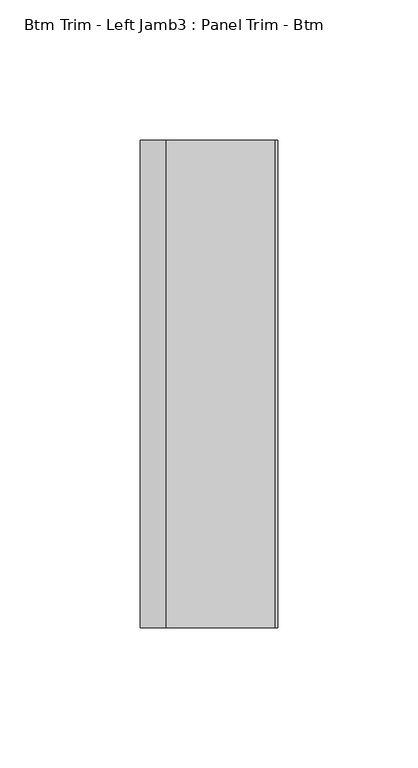
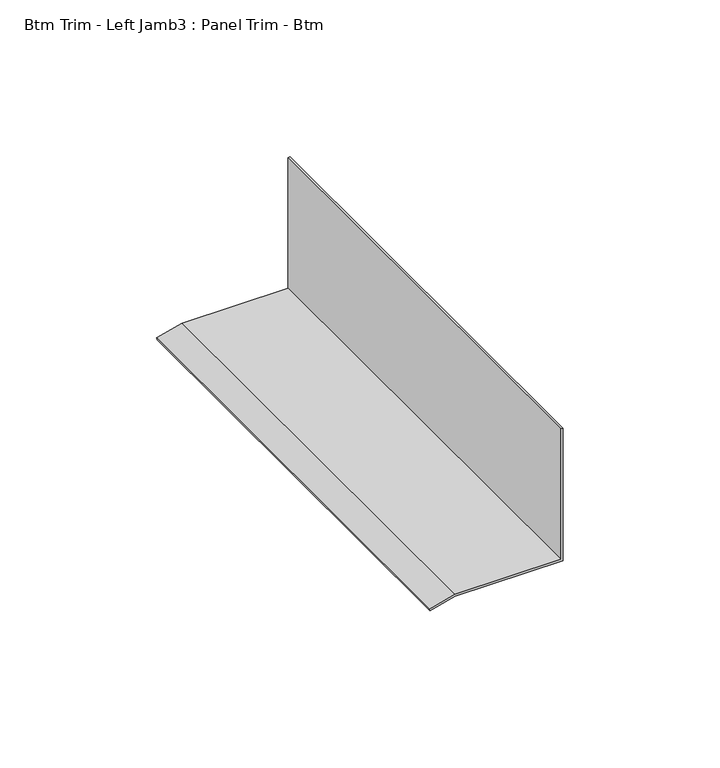
"""IFC4 building model written with IfcOpenShell, lengths in millimetres: proxy geometry, Btm Trim - Left Jamb3 : Panel Trim - Btm."""

from ifc_helpers import new_model, si_unit, frame, origin, place, context, project, spatial, polyline, outline, extrude, source, transform, mapped, element, save


def btm_trim_left_jamb3_panel_trim_btm_7869e14d(model_context):
    return source(origin(), model_context, "Body", "SweptSolid", [
        extrude(outline(polyline([(12.7, 587326.9015748), (10.2077022, 587317.6001928), (9.4409986, 587317.8056304), (11.90625, 587327.0060739), (11.90625, 587366.6808739), (63.5, 587366.6808739), (63.5, 587365.8934739), (12.7, 587365.8934739), (12.7, 587326.9015748)])), frame((0.0, -531775.7413841, 0.0), z_axis=(0.0, 1.0, 0.0), x_axis=(0.0, 0.0, 1.0)), (0.0, 0.0, 1.0), 174.0154),
    ])


if __name__ == "__main__":
    model = new_model("IFC4")
    model_context = context("Model", 3, world=origin())
    ifc_project = project(units=[si_unit("LENGTHUNIT", "METRE", prefix="MILLI")], contexts=[model_context])
    site = spatial("IfcSite", under=ifc_project)
    building = spatial("IfcBuilding", under=site)
    placement = place(None, origin())
    btm_trim_left_jamb3_panel_trim_btm_shape = btm_trim_left_jamb3_panel_trim_btm_7869e14d(model_context)
    element("IfcBuildingElementProxy", 1, Name="Btm Trim - Left Jamb3 : Panel Trim - Btm", ObjectType="Btm Trim - Left Jamb3 : Panel Trim - Btm", at=placement, inside=building, context=model_context, shape_type="MappedRepresentation", body=[
        mapped(btm_trim_left_jamb3_panel_trim_btm_shape, transform((0.0, 0.0, 0.0), x_axis=(1.0, 0.0, 0.0), y_axis=(0.0, 1.0, 0.0), z_axis=(0.0, 0.0, 1.0))),
    ])
    save(model, "model.ifc")

# Revit data of these elements
# Element 1 (IfcBuildingElementProxy, "Btm Trim - Left Jamb3 : Panel Trim - Btm")
#   Materials on its faces: "BASE TRIM BY MTL PANEL MFR."
# Materials
#   "BASE TRIM BY MTL PANEL MFR.": class "Generic", colour RGB 239 242 240, transparency 0, Cost = 0
